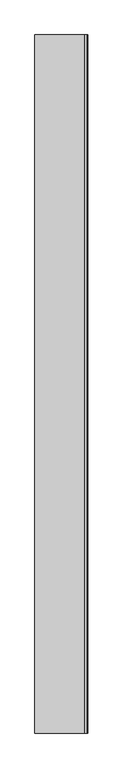
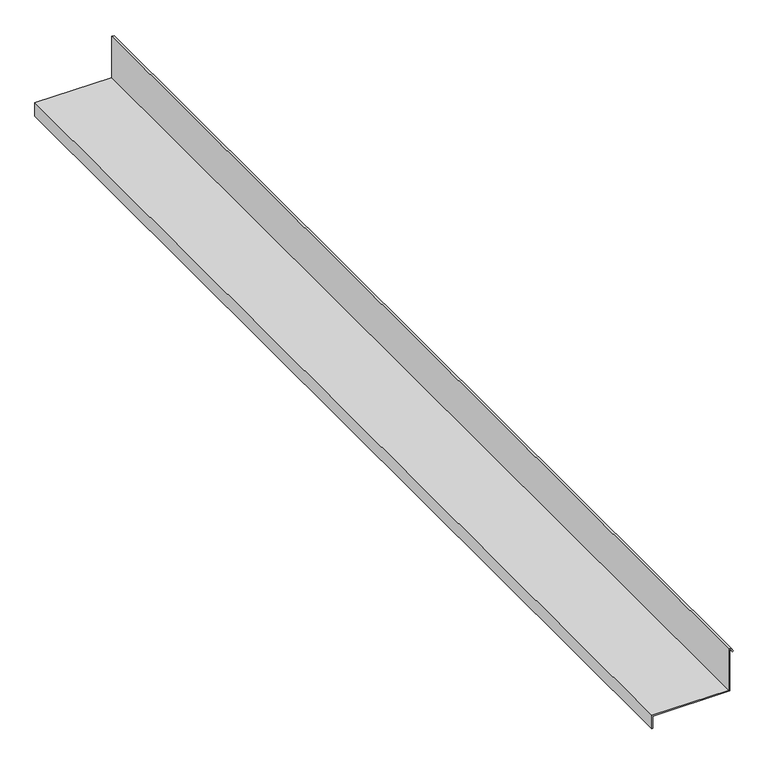
"""IFC4 building model written with IfcOpenShell, lengths in millimetres: proxy geometry, Flashing019 11084 : Flashing019 11084."""

from ifc_helpers import new_model, si_unit, frame, origin, place, context, project, spatial, polyline, outline, extrude, source, transform, mapped, element, save


def generic_models_9dc0ec64(model_context):
    return source(origin(), model_context, "Body", "SweptSolid", [
        extrude(outline(polyline([(40784.7382813, 16649.96875), (40784.7382813, 16645.2851562), (40703.2466161, 16645.2851562), (40703.2466161, 16501.84375), (40677.1179688, 16501.84375), (40677.1179688, 16503.84375), (40701.2466161, 16503.84375), (40701.2466161, 16647.2851563), (40782.7382813, 16647.2851563), (40782.7382813, 16648.7903893), (40776.8666698, 16652.0435345), (40777.8359375, 16653.7929687), (40784.7382813, 16649.96875)])), frame((0.0, 7982.1449366, 0.0), z_axis=(0.0, 1.0, 0.0), x_axis=(0.0, 0.0, 1.0)), (0.0, 0.0, 1.0), 2000.0),
    ])


if __name__ == "__main__":
    model = new_model("IFC4")
    model_context = context("Model", 3, world=origin())
    ifc_project = project(units=[si_unit("LENGTHUNIT", "METRE", prefix="MILLI")], contexts=[model_context])
    site = spatial("IfcSite", under=ifc_project)
    building = spatial("IfcBuilding", under=site)
    placement = place(None, origin())
    generic_models_shape = generic_models_9dc0ec64(model_context)
    element("IfcBuildingElementProxy", 1, Name="Flashing019 11084 : Flashing019 11084", ObjectType="Flashing019 11084 : Flashing019 11084", at=placement, inside=building, context=model_context, shape_type="MappedRepresentation", body=[
        mapped(generic_models_shape, transform((0.0, 0.0, 0.0), x_axis=(1.0, 0.0, 0.0), y_axis=(0.0, 1.0, 0.0), z_axis=(0.0, 0.0, 1.0))),
    ])
    save(model, "model.ifc")

# Revit data of these elements
# Type "Flashing019 11084 : Flashing019 11084"
#   NameOverride = "Flashing019"
# Element 1 (IfcBuildingElementProxy, "Flashing019 11084 : Flashing019 11084")
#   Materials on its faces: "BRAKE METAL FLASHING TO MATCH STOREFRONT"
# Materials
#   "BRAKE METAL FLASHING TO MATCH STOREFRONT": class "Unassigned", colour RGB 128 128 128, transparency 0
